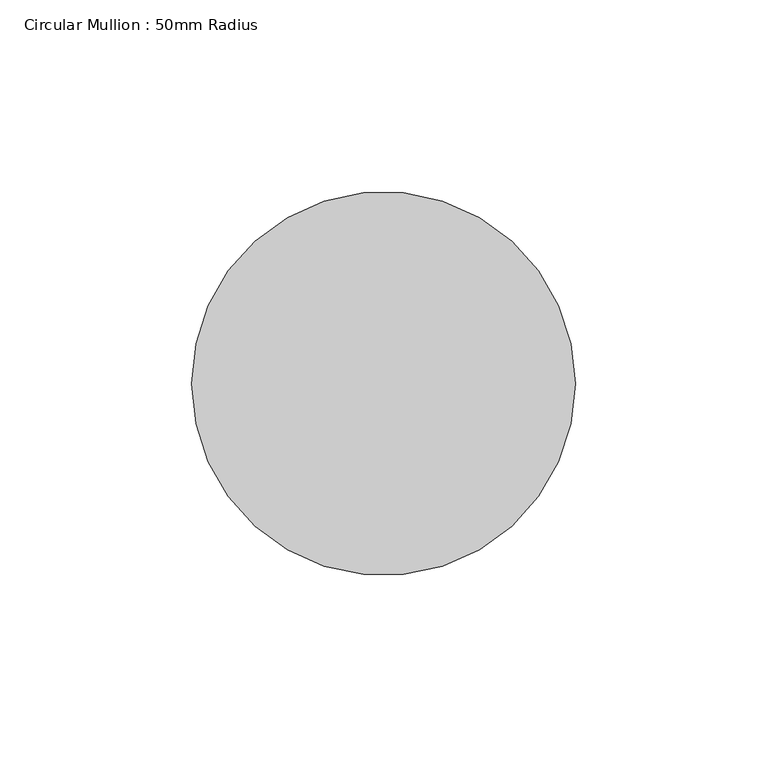
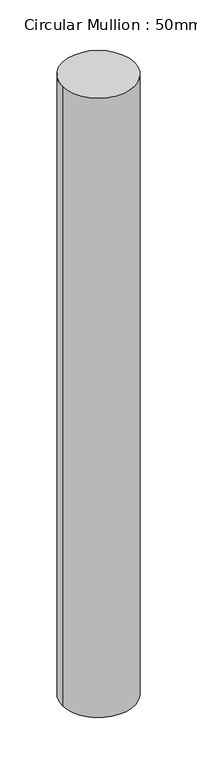
"""IFC4 building model written with IfcOpenShell, lengths in millimetres: member geometry, Circular Mullion : 50mm Radius."""

from ifc_helpers import new_model, si_unit, point, frame, origin, origin_2d, place, context, project, spatial, circle_curve, trimmed, segment, composite_curve, outline, extrude, source, transform, mapped, element, save


def circular_mullion_50mm_radius_3e5ce46e(model_context):
    return source(origin(), model_context, "Body", "SweptSolid", [
        extrude(outline(composite_curve([segment(trimmed(circle_curve(origin_2d(), 50.0), [point((50.0, 0.0))], [point((-50.0, 0.0))], False, "CARTESIAN"), True, "CONTINUOUS"), segment(trimmed(circle_curve(origin_2d(), 50.0), [point((-50.0, 0.0))], [point((50.0, 0.0))], False, "CARTESIAN"), True, "CONTINUOUS")], self_intersect=False)), frame((0.0, 0.0, -906.8229469), z_axis=(0.0, 0.0, 1.0), x_axis=(1.0, 0.0, 0.0)), (0.0, 0.0, 1.0), 906.8229469),
    ])


if __name__ == "__main__":
    model = new_model("IFC4")
    model_context = context("Model", 3, world=origin())
    ifc_project = project(units=[si_unit("LENGTHUNIT", "METRE", prefix="MILLI")], contexts=[model_context])
    site = spatial("IfcSite", under=ifc_project)
    building = spatial("IfcBuilding", under=site)
    placement = place(None, origin())
    circular_mullion_50mm_radius_shape = circular_mullion_50mm_radius_3e5ce46e(model_context)
    element("IfcMember", 1, ObjectType="Circular Mullion : 50mm Radius", at=placement, inside=building, context=model_context, shape_type="MappedRepresentation", body=[
        mapped(circular_mullion_50mm_radius_shape, transform((0.0, 0.0, 0.0), x_axis=(1.0, 0.0, 0.0), y_axis=(0.0, 1.0, 0.0), z_axis=(0.0, 0.0, 1.0))),
    ])
    save(model, "model.ifc")

# Revit data of these elements
# Type "Circular Mullion : 50mm Radius"
#   built-in parameter 1007350 = 0.164042 (stored number, unit not read)
# Element 1 (IfcMember, "Circular Mullion : 50mm Radius")
#   Materials on its faces: "Aluminium"
# Materials
#   "Aluminium": class "Metal", colour RGB 247 247 247, transparency 0, Description = "Aluminium 6061", Cost = 0
